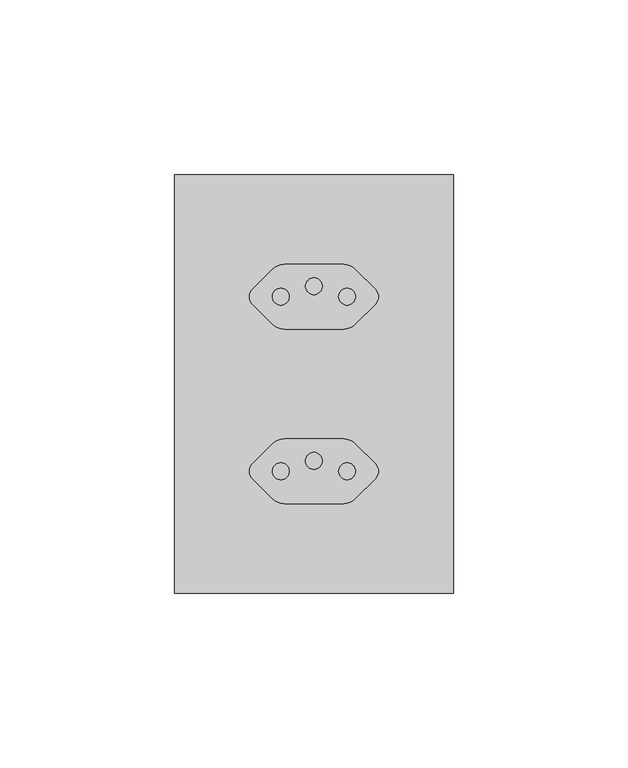
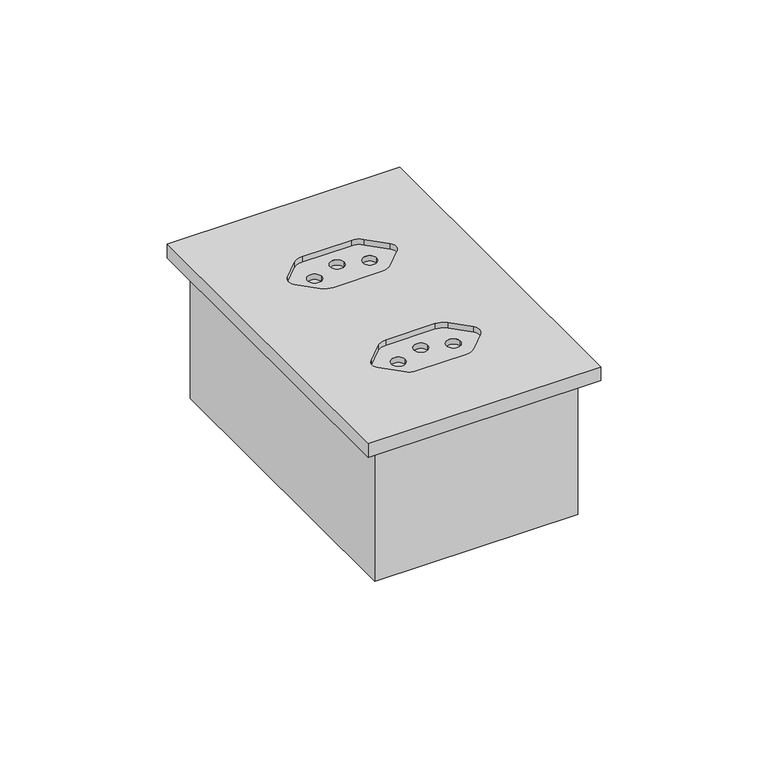
"""IFC4 building model written with IfcOpenShell, lengths in millimetres: proxy geometry, CAIXA VERTICE V7 : Tomada 20A 2s."""

from ifc_helpers import new_model, si_unit, frame, origin, place, context, project, spatial, polyline, circle_curve, faceted_brep, source, transform, mapped, element, save
from ifc_brep_helpers import plane_surface, revolved_surface, advanced_brep


def electrical_fixtures_352ae751(model_context):
    return source(origin(), model_context, "Body", "SolidModel", [
        faceted_brep([(33.0, 247.0, -48.0), (33.0, 353.0, -48.0), (-33.0, 353.0, -48.0), (-33.0, 247.0, -48.0), (35.0, 355.0, -50.0), (35.0, 245.0, -50.0), (-35.0, 245.0, -50.0), (-35.0, 355.0, -50.0), (-35.0, 355.0, 0.0), (35.0, 355.0, 0.0), (-35.0, 245.0, 0.0), (35.0, 245.0, 0.0), (33.0, 353.0, 0.0), (33.0, 247.0, 0.0), (-33.0, 247.0, 0.0), (-33.0, 353.0, 0.0)], [[[0, 1, 2, 3]], [[4, 5, 6, 7]], [[4, 7, 8, 9]], [[8, 7, 6, 10]], [[10, 6, 5, 11]], [[11, 5, 4, 9]], [[9, 8, 10, 11], [12, 13, 14, 15]], [[13, 12, 1, 0]], [[14, 13, 0, 3]], [[15, 14, 3, 2]], [[12, 15, 2, 1]]]),
        advanced_brep(
        [(40.0, 360.0, 5.0), (-40.0, 360.0, 5.0), (-40.0, 240.0, 5.0), (40.0, 240.0, 5.0), (8.4215729, 315.75, 5.0), (-8.4215729, 315.75, 5.0), (-11.9571068, 317.2144661, 5.0), (-17.6213203, 322.8786797, 5.0), (-17.6213203, 327.1213203, 5.0), (-11.9571068, 332.7855339, 5.0), (-8.4215729, 334.25, 5.0), (8.4215729, 334.25, 5.0), (11.9571068, 332.7855339, 5.0), (17.6213203, 327.1213203, 5.0), (17.6213203, 322.8786797, 5.0), (11.9571068, 317.2144661, 5.0), (8.4215729, 265.75, 5.0), (-8.4215729, 265.75, 5.0), (-11.9571068, 267.2144661, 5.0), (-17.6213203, 272.8786797, 5.0), (-17.6213203, 277.1213203, 5.0), (-11.9571068, 282.7855339, 5.0), (-8.4215729, 284.25, 5.0), (8.4215729, 284.25, 5.0), (11.9571068, 282.7855339, 5.0), (17.6213203, 277.1213203, 5.0), (17.6213203, 272.8786797, 5.0), (11.9571068, 267.2144661, 5.0), (-40.0, 360.0, 0.0), (40.0, 360.0, 0.0), (40.0, 240.0, 0.0), (-40.0, 240.0, 0.0), (8.4215729, 315.75, 3.0), (11.9571068, 317.2144661, 3.0), (17.6213203, 322.8786797, 3.0), (17.6213203, 327.1213203, 3.0), (11.9571068, 332.7855339, 3.0), (8.4215729, 334.25, 3.0), (-8.4215729, 334.25, 3.0), (-11.9571068, 332.7855339, 3.0), (-17.6213203, 327.1213203, 3.0), (-17.6213203, 322.8786797, 3.0), (-11.9571068, 317.2144661, 3.0), (-8.4215729, 315.75, 3.0), (-7.1, 325.0, 3.0), (-11.9, 325.0, 3.0), (11.9, 325.0, 3.0), (7.1, 325.0, 3.0), (2.4, 328.0, 3.0), (-2.4, 328.0, 3.0), (-11.9, 325.0, 1.0), (-7.1, 325.0, 1.0), (7.1, 325.0, 1.0), (11.9, 325.0, 1.0), (-2.4, 328.0, 1.0), (2.4, 328.0, 1.0), (8.4215729, 265.75, 3.0), (11.9571068, 267.2144661, 3.0), (17.6213203, 272.8786797, 3.0), (17.6213203, 277.1213203, 3.0), (11.9571068, 282.7855339, 3.0), (8.4215729, 284.25, 3.0), (-8.4215729, 284.25, 3.0), (-11.9571068, 282.7855339, 3.0), (-17.6213203, 277.1213203, 3.0), (-17.6213203, 272.8786797, 3.0), (-11.9571068, 267.2144661, 3.0), (-8.4215729, 265.75, 3.0), (-7.1, 275.0, 3.0), (-11.9, 275.0, 3.0), (11.9, 275.0, 3.0), (7.1, 275.0, 3.0), (2.4, 278.0, 3.0), (-2.4, 278.0, 3.0), (-11.9, 275.0, 1.0), (-7.1, 275.0, 1.0), (7.1, 275.0, 1.0), (11.9, 275.0, 1.0), (-2.4, 278.0, 1.0), (2.4, 278.0, 1.0)],
        [
            (0, 1),
            (1, 2),
            (2, 3),
            (3, 0),
            (4, 5),
            (5, 6, circle_curve(frame((-8.4215729, 320.75, 5.0), z_axis=(0.0, 0.0, -1.0), x_axis=(-1.0, 0.0, 0.0)), 5.0)),
            (6, 7),
            (7, 8, circle_curve(frame((-15.5, 325.0, 5.0), z_axis=(0.0, 0.0, -1.0), x_axis=(-1.0, 0.0, 0.0)), 3.0)),
            (8, 9),
            (9, 10, circle_curve(frame((-8.4215729, 329.25, 5.0), z_axis=(0.0, 0.0, -1.0), x_axis=(-1.0, 0.0, 0.0)), 5.0)),
            (10, 11),
            (11, 12, circle_curve(frame((8.4215729, 329.25, 5.0), z_axis=(0.0, 0.0, -1.0), x_axis=(-1.0, 0.0, 0.0)), 5.0)),
            (12, 13),
            (13, 14, circle_curve(frame((15.5, 325.0, 5.0), z_axis=(0.0, 0.0, -1.0), x_axis=(-1.0, 0.0, 0.0)), 3.0)),
            (14, 15),
            (15, 4, circle_curve(frame((8.4215729, 320.75, 5.0), z_axis=(0.0, 0.0, -1.0), x_axis=(-1.0, 0.0, 0.0)), 5.0)),
            (16, 17),
            (17, 18, circle_curve(frame((-8.4215729, 270.75, 5.0), z_axis=(0.0, 0.0, -1.0), x_axis=(-1.0, 0.0, 0.0)), 5.0)),
            (18, 19),
            (19, 20, circle_curve(frame((-15.5, 275.0, 5.0), z_axis=(0.0, 0.0, -1.0), x_axis=(-1.0, 0.0, 0.0)), 3.0)),
            (20, 21),
            (21, 22, circle_curve(frame((-8.4215729, 279.25, 5.0), z_axis=(0.0, 0.0, -1.0), x_axis=(-1.0, 0.0, 0.0)), 5.0)),
            (22, 23),
            (23, 24, circle_curve(frame((8.4215729, 279.25, 5.0), z_axis=(0.0, 0.0, -1.0), x_axis=(-1.0, 0.0, 0.0)), 5.0)),
            (24, 25),
            (25, 26, circle_curve(frame((15.5, 275.0, 5.0), z_axis=(0.0, 0.0, -1.0), x_axis=(-1.0, 0.0, 0.0)), 3.0)),
            (26, 27),
            (27, 16, circle_curve(frame((8.4215729, 270.75, 5.0), z_axis=(0.0, 0.0, -1.0), x_axis=(-1.0, 0.0, 0.0)), 5.0)),
            (28, 29),
            (29, 30),
            (30, 31),
            (31, 28),
            (0, 29),
            (28, 1),
            (31, 2),
            (30, 3),
            (32, 33, circle_curve(frame((8.4215729, 320.75, 3.0), z_axis=(0.0, 0.0, 1.0), x_axis=(-1.0, 0.0, 0.0)), 5.0)),
            (33, 34),
            (34, 35, circle_curve(frame((15.5, 325.0, 3.0), z_axis=(0.0, 0.0, 1.0), x_axis=(-1.0, 0.0, 0.0)), 3.0)),
            (35, 36),
            (36, 37, circle_curve(frame((8.4215729, 329.25, 3.0), z_axis=(0.0, 0.0, 1.0), x_axis=(-1.0, 0.0, 0.0)), 5.0)),
            (37, 38),
            (38, 39, circle_curve(frame((-8.4215729, 329.25, 3.0), z_axis=(0.0, 0.0, 1.0), x_axis=(-1.0, 0.0, 0.0)), 5.0)),
            (39, 40),
            (40, 41, circle_curve(frame((-15.5, 325.0, 3.0), z_axis=(0.0, 0.0, 1.0), x_axis=(-1.0, 0.0, 0.0)), 3.0)),
            (41, 42),
            (42, 43, circle_curve(frame((-8.4215729, 320.75, 3.0), z_axis=(0.0, 0.0, 1.0), x_axis=(-1.0, 0.0, 0.0)), 5.0)),
            (43, 32),
            (44, 45, circle_curve(frame((-9.5, 325.0, 3.0), z_axis=(0.0, 0.0, -1.0), x_axis=(1.0, 2.301812013077709e-12, 0.0)), 2.4)),
            (45, 44, circle_curve(frame((-9.5, 325.0, 3.0), z_axis=(0.0, 0.0, -1.0), x_axis=(1.0, 2.301812013077709e-12, 0.0)), 2.4)),
            (46, 47, circle_curve(frame((9.5, 325.0, 3.0), z_axis=(0.0, 0.0, -1.0), x_axis=(1.0, 2.301812013077709e-12, 0.0)), 2.4)),
            (47, 46, circle_curve(frame((9.5, 325.0, 3.0), z_axis=(0.0, 0.0, -1.0), x_axis=(1.0, 2.301812013077709e-12, 0.0)), 2.4)),
            (48, 49, circle_curve(frame((0.0, 328.0, 3.0), z_axis=(0.0, 0.0, -1.0), x_axis=(1.0, 2.301812013077709e-12, 0.0)), 2.4)),
            (49, 48, circle_curve(frame((0.0, 328.0, 3.0), z_axis=(0.0, 0.0, -1.0), x_axis=(1.0, 2.301812013077709e-12, 0.0)), 2.4)),
            (43, 5),
            (4, 32),
            (42, 6),
            (41, 7),
            (40, 8),
            (39, 9),
            (38, 10),
            (37, 11),
            (36, 12),
            (35, 13),
            (34, 14),
            (33, 15),
            (50, 51, circle_curve(frame((-9.5, 325.0, 1.0), z_axis=(0.0, 0.0, 1.0), x_axis=(1.0, 2.301812013077709e-12, 0.0)), 2.4)),
            (51, 50, circle_curve(frame((-9.5, 325.0, 1.0), z_axis=(0.0, 0.0, 1.0), x_axis=(1.0, 2.301812013077709e-12, 0.0)), 2.4)),
            (52, 53, circle_curve(frame((9.5, 325.0, 1.0), z_axis=(0.0, 0.0, 1.0), x_axis=(1.0, 2.301812013077709e-12, 0.0)), 2.4)),
            (53, 52, circle_curve(frame((9.5, 325.0, 1.0), z_axis=(0.0, 0.0, 1.0), x_axis=(1.0, 2.301812013077709e-12, 0.0)), 2.4)),
            (54, 55, circle_curve(frame((0.0, 328.0, 1.0), z_axis=(0.0, 0.0, 1.0), x_axis=(1.0, 2.301812013077709e-12, 0.0)), 2.4)),
            (55, 54, circle_curve(frame((0.0, 328.0, 1.0), z_axis=(0.0, 0.0, 1.0), x_axis=(1.0, 2.301812013077709e-12, 0.0)), 2.4)),
            (44, 51),
            (50, 45),
            (46, 53),
            (52, 47),
            (48, 55),
            (54, 49),
            (56, 57, circle_curve(frame((8.4215729, 270.75, 3.0), z_axis=(0.0, 0.0, 1.0), x_axis=(-1.0, 0.0, 0.0)), 5.0)),
            (57, 58),
            (58, 59, circle_curve(frame((15.5, 275.0, 3.0), z_axis=(0.0, 0.0, 1.0), x_axis=(-1.0, 0.0, 0.0)), 3.0)),
            (59, 60),
            (60, 61, circle_curve(frame((8.4215729, 279.25, 3.0), z_axis=(0.0, 0.0, 1.0), x_axis=(-1.0, 0.0, 0.0)), 5.0)),
            (61, 62),
            (62, 63, circle_curve(frame((-8.4215729, 279.25, 3.0), z_axis=(0.0, 0.0, 1.0), x_axis=(-1.0, 0.0, 0.0)), 5.0)),
            (63, 64),
            (64, 65, circle_curve(frame((-15.5, 275.0, 3.0), z_axis=(0.0, 0.0, 1.0), x_axis=(-1.0, 0.0, 0.0)), 3.0)),
            (65, 66),
            (66, 67, circle_curve(frame((-8.4215729, 270.75, 3.0), z_axis=(0.0, 0.0, 1.0), x_axis=(-1.0, 0.0, 0.0)), 5.0)),
            (67, 56),
            (68, 69, circle_curve(frame((-9.5, 275.0, 3.0), z_axis=(0.0, 0.0, -1.0), x_axis=(1.0, 2.301812013077709e-12, 0.0)), 2.4)),
            (69, 68, circle_curve(frame((-9.5, 275.0, 3.0), z_axis=(0.0, 0.0, -1.0), x_axis=(1.0, 2.301812013077709e-12, 0.0)), 2.4)),
            (70, 71, circle_curve(frame((9.5, 275.0, 3.0), z_axis=(0.0, 0.0, -1.0), x_axis=(1.0, 2.301812013077709e-12, 0.0)), 2.4)),
            (71, 70, circle_curve(frame((9.5, 275.0, 3.0), z_axis=(0.0, 0.0, -1.0), x_axis=(1.0, 2.301812013077709e-12, 0.0)), 2.4)),
            (72, 73, circle_curve(frame((0.0, 278.0, 3.0), z_axis=(0.0, 0.0, -1.0), x_axis=(1.0, 2.301812013077709e-12, 0.0)), 2.4)),
            (73, 72, circle_curve(frame((0.0, 278.0, 3.0), z_axis=(0.0, 0.0, -1.0), x_axis=(1.0, 2.301812013077709e-12, 0.0)), 2.4)),
            (67, 17),
            (16, 56),
            (66, 18),
            (65, 19),
            (64, 20),
            (63, 21),
            (62, 22),
            (61, 23),
            (60, 24),
            (59, 25),
            (58, 26),
            (57, 27),
            (74, 75, circle_curve(frame((-9.5, 275.0, 1.0), z_axis=(0.0, 0.0, 1.0), x_axis=(1.0, 2.301812013077709e-12, 0.0)), 2.4)),
            (75, 74, circle_curve(frame((-9.5, 275.0, 1.0), z_axis=(0.0, 0.0, 1.0), x_axis=(1.0, 2.301812013077709e-12, 0.0)), 2.4)),
            (76, 77, circle_curve(frame((9.5, 275.0, 1.0), z_axis=(0.0, 0.0, 1.0), x_axis=(1.0, 2.301812013077709e-12, 0.0)), 2.4)),
            (77, 76, circle_curve(frame((9.5, 275.0, 1.0), z_axis=(0.0, 0.0, 1.0), x_axis=(1.0, 2.301812013077709e-12, 0.0)), 2.4)),
            (78, 79, circle_curve(frame((0.0, 278.0, 1.0), z_axis=(0.0, 0.0, 1.0), x_axis=(1.0, 2.301812013077709e-12, 0.0)), 2.4)),
            (79, 78, circle_curve(frame((0.0, 278.0, 1.0), z_axis=(0.0, 0.0, 1.0), x_axis=(1.0, 2.301812013077709e-12, 0.0)), 2.4)),
            (68, 75),
            (74, 69),
            (70, 77),
            (76, 71),
            (72, 79),
            (78, 73),
        ],
        [
            plane_surface(frame((-60.0, 360.0, 5.0), z_axis=(0.0, 0.0, 1.0), x_axis=(-1.0, 0.0, 0.0))),
            plane_surface(frame((-60.0, 360.0, 0.0), z_axis=(0.0, 0.0, -1.0), x_axis=(1.0, 0.0, 0.0))),
            plane_surface(frame((40.0, 360.0, 5.0), z_axis=(0.0, 1.0, 0.0), x_axis=(0.0, 0.0, -1.0))),
            plane_surface(frame((-40.0, 360.0, 5.0), z_axis=(-1.0, 0.0, 0.0), x_axis=(0.0, 0.0, -1.0))),
            plane_surface(frame((-40.0, 240.0, 5.0), z_axis=(0.0, -1.0, 0.0), x_axis=(0.0, 0.0, -1.0))),
            plane_surface(frame((40.0, 240.0, 5.0), z_axis=(1.0, 0.0, 0.0), x_axis=(0.0, 0.0, -1.0))),
            plane_surface(frame((3.4215729, 320.75, 3.0), z_axis=(0.0, 0.0, 1.0), x_axis=(0.0, 1.0, 0.0))),
            plane_surface(frame((-8.4215729, 315.75, 5.0), z_axis=(0.0, 1.0, 0.0), x_axis=(0.0, 0.0, -1.0))),
            revolved_surface(polyline([(-13.4215729, 320.75, 5.0), (-13.4215729, 320.75, 3.0)]), (-8.4215729, 320.75, 3.0), (0.0, 0.0, 1.0)),
            plane_surface(frame((-17.6213203, 322.8786797, 5.0), z_axis=(0.7071067811865045, 0.7071067811865905, 0.0), x_axis=(0.0, 0.0, -1.0))),
            revolved_surface(polyline([(-18.5, 325.0, 5.0), (-18.5, 325.0, 3.0)]), (-15.5, 325.0, 3.0), (0.0, 0.0, 1.0)),
            plane_surface(frame((-11.9571068, 332.7855339, 5.0), z_axis=(0.7071067811865515, -0.7071067811865437, 0.0), x_axis=(0.0, 0.0, -1.0))),
            revolved_surface(polyline([(-13.4215729, 329.25, 5.0), (-13.4215729, 329.25, 3.0)]), (-8.4215729, 329.25, 3.0), (0.0, 0.0, 1.0)),
            plane_surface(frame((8.4215729, 334.25, 5.0), z_axis=(0.0, -1.0, 0.0), x_axis=(0.0, 0.0, -1.0))),
            revolved_surface(polyline([(3.4215728999999993, 329.25, 5.0), (3.4215728999999993, 329.25, 3.0)]), (8.4215729, 329.25, 3.0), (0.0, 0.0, 1.0)),
            plane_surface(frame((17.6213203, 327.1213203, 5.0), z_axis=(-0.7071067811865307, -0.7071067811865643, 0.0), x_axis=(0.0, 0.0, -1.0))),
            revolved_surface(polyline([(12.5, 325.0, 5.0), (12.5, 325.0, 3.0)]), (15.5, 325.0, 3.0), (0.0, 0.0, 1.0)),
            plane_surface(frame((11.9571068, 317.2144661, 5.0), z_axis=(-0.7071067811865893, 0.7071067811865058, 0.0), x_axis=(0.0, 0.0, -1.0))),
            revolved_surface(polyline([(3.4215728999999993, 320.75, 5.0), (3.4215728999999993, 320.75, 3.0)]), (8.4215729, 320.75, 3.0), (0.0, 0.0, 1.0)),
            plane_surface(frame((-7.1, 325.0, 1.0), z_axis=(0.0, 0.0, 1.0), x_axis=(2.301812013077709e-12, -1.0, 0.0))),
            revolved_surface(polyline([(-7.1, 325.0000000000055, 3.0), (-7.1, 325.0000000000055, 1.0)]), (-9.5, 325.0, 1.0), (0.0, 0.0, 1.0)),
            revolved_surface(polyline([(11.9, 325.0000000000055, 3.0), (11.9, 325.0000000000055, 1.0)]), (9.5, 325.0, 5.0), (0.0, 0.0, 1.0)),
            revolved_surface(polyline([(2.4, 328.0000000000055, 3.0), (2.4, 328.0000000000055, 1.0)]), (0.0, 328.0, 5.0), (0.0, 0.0, 1.0)),
            plane_surface(frame((3.4215729, 270.75, 3.0), z_axis=(0.0, 0.0, 1.0), x_axis=(0.0, 1.0, 0.0))),
            plane_surface(frame((-8.4215729, 265.75, 5.0), z_axis=(0.0, 1.0, 0.0), x_axis=(0.0, 0.0, -1.0))),
            revolved_surface(polyline([(-13.4215729, 270.75, 5.0), (-13.4215729, 270.75, 3.0)]), (-8.4215729, 270.75, 3.0), (0.0, 0.0, 1.0)),
            plane_surface(frame((-17.6213203, 272.8786797, 5.0), z_axis=(0.7071067811865045, 0.7071067811865905, 0.0), x_axis=(0.0, 0.0, -1.0))),
            revolved_surface(polyline([(-18.5, 275.0, 5.0), (-18.5, 275.0, 3.0)]), (-15.5, 275.0, 3.0), (0.0, 0.0, 1.0)),
            plane_surface(frame((-11.9571068, 282.7855339, 5.0), z_axis=(0.7071067811865515, -0.7071067811865437, 0.0), x_axis=(0.0, 0.0, -1.0))),
            revolved_surface(polyline([(-13.4215729, 279.25, 5.0), (-13.4215729, 279.25, 3.0)]), (-8.4215729, 279.25, 3.0), (0.0, 0.0, 1.0)),
            plane_surface(frame((8.4215729, 284.25, 5.0), z_axis=(0.0, -1.0, 0.0), x_axis=(0.0, 0.0, -1.0))),
            revolved_surface(polyline([(3.4215728999999993, 279.25, 5.0), (3.4215728999999993, 279.25, 3.0)]), (8.4215729, 279.25, 3.0), (0.0, 0.0, 1.0)),
            plane_surface(frame((17.6213203, 277.1213203, 5.0), z_axis=(-0.7071067811865307, -0.7071067811865643, 0.0), x_axis=(0.0, 0.0, -1.0))),
            revolved_surface(polyline([(12.5, 275.0, 5.0), (12.5, 275.0, 3.0)]), (15.5, 275.0, 3.0), (0.0, 0.0, 1.0)),
            plane_surface(frame((11.9571068, 267.2144661, 5.0), z_axis=(-0.7071067811865893, 0.7071067811865058, 0.0), x_axis=(0.0, 0.0, -1.0))),
            revolved_surface(polyline([(3.4215728999999993, 270.75, 5.0), (3.4215728999999993, 270.75, 3.0)]), (8.4215729, 270.75, 3.0), (0.0, 0.0, 1.0)),
            plane_surface(frame((-7.1, 275.0, 1.0), z_axis=(0.0, 0.0, 1.0), x_axis=(2.301812013077709e-12, -1.0, 0.0))),
            revolved_surface(polyline([(-7.1, 275.0000000000055, 3.0), (-7.1, 275.0000000000055, 1.0)]), (-9.5, 275.0, 1.0), (0.0, 0.0, 1.0)),
            revolved_surface(polyline([(11.9, 275.0000000000055, 3.0), (11.9, 275.0000000000055, 1.0)]), (9.5, 275.0, 5.0), (0.0, 0.0, 1.0)),
            revolved_surface(polyline([(2.4, 278.0000000000055, 3.0), (2.4, 278.0000000000055, 1.0)]), (0.0, 278.0, 5.0), (0.0, 0.0, 1.0)),
        ],
        [
            (0, [[1, 2, 3, 4], [5, 6, 7, 8, 9, 10, 11, 12, 13, 14, 15, 16], [17, 18, 19, 20, 21, 22, 23, 24, 25, 26, 27, 28]]),
            (1, [[29, 30, 31, 32]]),
            (2, [[-1, 33, -29, 34]]),
            (3, [[-2, -34, -32, 35]]),
            (4, [[-3, -35, -31, 36]]),
            (5, [[-4, -36, -30, -33]]),
            (6, [[37, 38, 39, 40, 41, 42, 43, 44, 45, 46, 47, 48], [49, 50], [51, 52], [53, 54]]),
            (7, [[-48, 55, -5, 56]]),
            (8, [[-47, 57, -6, -55]]),
            (9, [[-46, 58, -7, -57]]),
            (10, [[-45, 59, -8, -58]]),
            (11, [[-44, 60, -9, -59]]),
            (12, [[-43, 61, -10, -60]]),
            (13, [[-42, 62, -11, -61]]),
            (14, [[-41, 63, -12, -62]]),
            (15, [[-40, 64, -13, -63]]),
            (16, [[-39, 65, -14, -64]]),
            (17, [[-38, 66, -15, -65]]),
            (18, [[-37, -56, -16, -66]]),
            (19, [[67, 68]]),
            (19, [[69, 70]]),
            (19, [[71, 72]]),
            (20, [[-49, 73, -67, 74]]),
            (20, [[-50, -74, -68, -73]]),
            (21, [[-51, 75, -69, 76]]),
            (21, [[-52, -76, -70, -75]]),
            (22, [[-53, 77, -71, 78]]),
            (22, [[-54, -78, -72, -77]]),
            (23, [[79, 80, 81, 82, 83, 84, 85, 86, 87, 88, 89, 90], [91, 92], [93, 94], [95, 96]]),
            (24, [[-90, 97, -17, 98]]),
            (25, [[-89, 99, -18, -97]]),
            (26, [[-88, 100, -19, -99]]),
            (27, [[-87, 101, -20, -100]]),
            (28, [[-86, 102, -21, -101]]),
            (29, [[-85, 103, -22, -102]]),
            (30, [[-84, 104, -23, -103]]),
            (31, [[-83, 105, -24, -104]]),
            (32, [[-82, 106, -25, -105]]),
            (33, [[-81, 107, -26, -106]]),
            (34, [[-80, 108, -27, -107]]),
            (35, [[-79, -98, -28, -108]]),
            (36, [[109, 110]]),
            (36, [[111, 112]]),
            (36, [[113, 114]]),
            (37, [[-91, 115, -109, 116]]),
            (37, [[-92, -116, -110, -115]]),
            (38, [[-93, 117, -111, 118]]),
            (38, [[-94, -118, -112, -117]]),
            (39, [[-95, 119, -113, 120]]),
            (39, [[-96, -120, -114, -119]]),
        ],
    ),
    ])


if __name__ == "__main__":
    model = new_model("IFC4")
    model_context = context("Model", 3, world=origin())
    ifc_project = project(units=[si_unit("LENGTHUNIT", "METRE", prefix="MILLI")], contexts=[model_context])
    site = spatial("IfcSite", under=ifc_project)
    building = spatial("IfcBuilding", under=site)
    placement = place(None, origin())
    electrical_fixtures_shape = electrical_fixtures_352ae751(model_context)
    element("IfcBuildingElementProxy", 1, Name="CAIXA VERTICE V7 : Tomada 20A 2s", ObjectType="CAIXA VERTICE V7 : Tomada 20A 2s", at=placement, inside=building, context=model_context, shape_type="MappedRepresentation", body=[
        mapped(electrical_fixtures_shape, transform((0.0, 0.0, 0.0), x_axis=(1.0, 0.0, 0.0), y_axis=(0.0, 1.0, 0.0), z_axis=(0.0, 0.0, 1.0))),
    ])
    save(model, "model.ifc")

# Revit data of these elements
# Type "CAIXA VERTICE V7 : Tomada 20A 2s"
#   URL = "www.facebook.com/verticetreinamentos"
#   SEÇÃO [instance default] = ""
#   Rotação [instance default] = 0.00°
#   LARGURA DA TAMPA = 0.08 m
#   BORDA = 0.01 m
#   ALTURA DE INSTALAÇÃO [instance default] = 1.10 m
#   Distância Anotação [instance default] = 0.0015 m
#   ALTURA DA TAMPA = 0.12 m
#   Vertical [instance default] = yes
#   VER SEÇÃO [instance default] = no
#   SHADE ESQ [instance default] = no
#   SHADE DIR [instance default] = yes
#   HORIZONTAL [instance default] = no
#   ANDAR COM A LEGENDA [instance default] = 0
#   Material Tampa [instance default] = Plástico, branco opaco
#   Caixa = element 1798518
#   Anotação = element 1798532
#   Default Elevation = 0
# Element 1 (IfcBuildingElementProxy, "CAIXA VERTICE V7 : Tomada 20A 2s")
#   ALTURA DE INSTALAÇÃO = 0.30 m
#   SHADE DIR = no
#   Materials on its faces: "Plástico, branco opaco"
# Materials
#   "Plástico, branco opaco": class "Plástico", colour RGB 120 120 120, transparency 0, Description = "Plastic, generic, opaque white", Cost = 0
